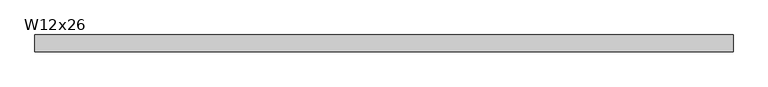
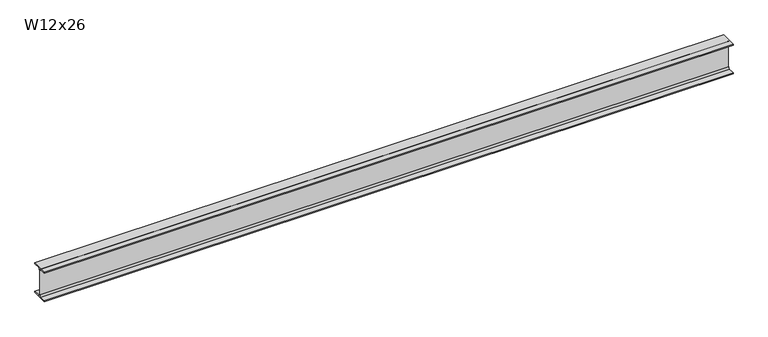
"""IFC4 building model written with IfcOpenShell, lengths in millimetres: beam geometry, RME W-Wide Flange : W12x26."""

from ifc_helpers import new_model, si_unit, point, frame, frame_2d, origin, place, context, project, spatial, polyline, circle_curve, trimmed, segment, composite_curve, outline, extrude, source, transform, mapped, element, save


def w12x26_5a31e400(model_context):
    return source(origin(), model_context, "Body", "SweptSolid", [
        extrude(outline(composite_curve([segment(polyline([(82.423, -145.288), (82.423, -154.94), (-82.423, -154.94), (-82.423, -145.288), (-20.2565, -145.288)]), True, "CONTINUOUS"), segment(trimmed(circle_curve(frame_2d((-20.2565, -127.9525)), 17.3355), [point((-20.2565, -145.288))], [point((-2.921, -127.9525))], True, "CARTESIAN"), True, "CONTINUOUS"), segment(polyline([(-2.921, -127.9525), (-2.921, 127.9525)]), True, "CONTINUOUS"), segment(trimmed(circle_curve(frame_2d((-20.2565, 127.9525)), 17.3355), [point((-2.921, 127.9525))], [point((-20.2565, 145.288))], True, "CARTESIAN"), True, "CONTINUOUS"), segment(polyline([(-20.2565, 145.288), (-82.423, 145.288), (-82.423, 154.94), (82.423, 154.94), (82.423, 145.288), (20.2565, 145.288)]), True, "CONTINUOUS"), segment(trimmed(circle_curve(frame_2d((20.2565, 127.9525)), 17.3355), [point((20.2565, 145.288))], [point((2.921, 127.9525))], True, "CARTESIAN"), True, "CONTINUOUS"), segment(polyline([(2.921, 127.9525), (2.921, -127.9525)]), True, "CONTINUOUS"), segment(trimmed(circle_curve(frame_2d((20.2565, -127.9525)), 17.3355), [point((2.921, -127.9525))], [point((20.2565, -145.288))], True, "CARTESIAN"), True, "CONTINUOUS"), segment(polyline([(20.2565, -145.288), (82.423, -145.288)]), True, "CONTINUOUS")], self_intersect=False)), frame((-3251.7186122, 0.0, 0.0), z_axis=(1.0, 0.0, 0.0), x_axis=(0.0, 1.0, 0.0)), (0.0, 0.0, 1.0), 6876.7442954),
    ])


if __name__ == "__main__":
    model = new_model("IFC4")
    model_context = context("Model", 3, world=origin())
    ifc_project = project(units=[si_unit("LENGTHUNIT", "METRE", prefix="MILLI")], contexts=[model_context])
    site = spatial("IfcSite", under=ifc_project)
    building = spatial("IfcBuilding", under=site)
    placement = place(None, origin())
    w12x26_shape = w12x26_5a31e400(model_context)
    element("IfcBeam", 1, ObjectType="RME W-Wide Flange : W12x26", at=placement, inside=building, context=model_context, shape_type="MappedRepresentation", body=[
        mapped(w12x26_shape, transform((0.0, 0.0, 0.0), x_axis=(1.0, 0.0, 0.0), y_axis=(0.0, 1.0, 0.0), z_axis=(0.0, 0.0, 1.0))),
    ])
    save(model, "model.ifc")

# Revit data of these elements
# Type "RME W-Wide Flange : W12x26"
#   WELD P [instance default] = ""
#   WELD LE [instance default] = ""
#   WELD D [instance default] = ""
#   TOP SECTION SIZE [instance default] = ""
#   TOP SECTION LENGTH [instance default] = ""
#   REMARKS [instance default] = ""
#   REINF TYPE [instance default] = ""
#   Nominal Size = "W24"
#   End Bearing Capacity [instance default] = ""
#   BOT SECTION SIZE [instance default] = ""
#   BOT SECTION LENGTH [instance default] = ""
#   Assembly Code = "B10"
#   W = 26
#   Start Extension Calculation [instance default] = 10' - 0"
#   Start Extension [instance default] = -0' - 0 1/2"
#   End Extension Calculation [instance default] = 10' - 0"
#   End Extension [instance default] = -0' - 0 1/2"
#   Length [instance default] = 5' - 0"
#   bf = 0' - 6.49"
#   d = 1' - 0.2"
#   k = 0' - 1 1/16"
#   k2 = 0' - 0.6825"
#   tf = 0' - 0.38"
#   tw = 0' - 0.23"
#   A = 0.053125 SF
#   Structural Material [instance default] = Metal - Steel - ASTM A992
# Element 1 (IfcBeam, "RME W-Wide Flange : W12x26")
#   Start Extension Calculation = 11' - 4.69574"
#   Start Extension = 1' - 4.19574"
#   End Extension Calculation = 10' - 9 1/8"
#   End Extension = 0' - 8 5/8"
#   Length = 21' - 7.8101"
#   Materials on its faces: "Metal - Steel - ASTM A992"
# Materials
#   "Metal - Steel - ASTM A992": class "Metal", colour RGB 255 128 0, transparency 0
